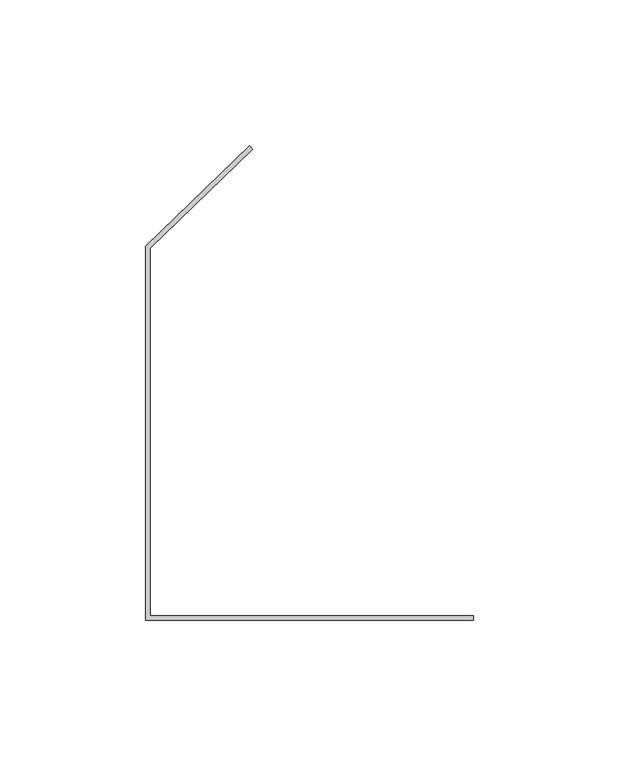
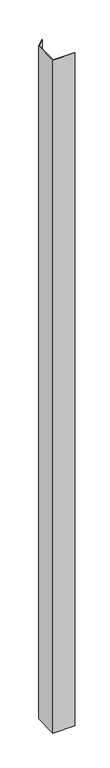
"""IFC4 building model written with IfcOpenShell, lengths in millimetres: proxy geometry, Generic Models 11:Generic Models 1:306267:Generic Models 1:306267 : Generic Models 11:Generic Models 1:306267:300405:Generic Models 1:306267:Generic Models 1:306267 : Generic Models 11:Generic Models 1:306267:300405 : Generic Models 11:Generic Models 1:306267:Generic Models 1:306267 : Generic Models 11:Generic Models 1:306267:300405:22 : Generic Models 11:Generic Models 1:306267:Generic Models 1:306267 : Generic Models 11:Generic Models 1:306267:300405:Generic Models 1:306267:Generic Models 1:306267 : Generic Models 11:Generic Models 1:306267:300405 : Generic Models 11:Generic Models 1:306267:Generic Models 1:306267 : Generic Models 11:Generic Models 1:306267:300405:300182."""

from ifc_helpers import new_model, si_unit, frame, origin, place, context, project, spatial, polyline, outline, extrude, source, transform, mapped, element, save


def generic_models_ad167b78(model_context):
    return source(origin(), model_context, "Body", "SweptSolid", [
        extrude(outline(polyline([(578579.828326, -568246.7263189), (578579.828326, -568118.5331318), (578615.3859082, -568084.0659821), (578616.5085764, -568085.1886502), (578581.415826, -568119.2052228), (578581.415826, -568245.1388189), (578692.2171387, -568245.1388189), (578692.2171387, -568246.7263189), (578579.828326, -568246.7263189)])), frame((0.0, 0.0, 4853.797603), z_axis=(0.0, 0.0, 1.0), x_axis=(1.0, 0.0, 0.0)), (0.0, 0.0, 1.0), 3695.7),
    ])


if __name__ == "__main__":
    model = new_model("IFC4")
    model_context = context("Model", 3, world=origin())
    ifc_project = project(units=[si_unit("LENGTHUNIT", "METRE", prefix="MILLI")], contexts=[model_context])
    site = spatial("IfcSite", under=ifc_project)
    building = spatial("IfcBuilding", under=site)
    placement = place(None, origin())
    generic_models_shape = generic_models_ad167b78(model_context)
    element("IfcBuildingElementProxy", 1, Name="Generic Models 11:Generic Models 1:306267:Generic Models 1:306267 : Generic Models 11:Generic Models 1:306267:300405:Generic Models 1:306267:Generic Models 1:306267 : Generic Models 11:Generic Models 1:306267:300405 : Generic Models 11:Generic Models 1:306267:Generic Models 1:306267 : Generic Models 11:Generic Models 1:306267:300405:22 : Generic Models 11:Generic Models 1:306267:Generic Models 1:306267 : Generic Models 11:Generic Models 1:306267:300405:Generic Models 1:306267:Generic Models 1:306267 : Generic Models 11:Generic Models 1:306267:300405 : Generic Models 11:Generic Models 1:306267:Generic Models 1:306267 : Generic Models 11:Generic Models 1:306267:300405:300182", ObjectType="Generic Models 11:Generic Models 1:306267:Generic Models 1:306267 : Generic Models 11:Generic Models 1:306267:300405:Generic Models 1:306267:Generic Models 1:306267 : Generic Models 11:Generic Models 1:306267:300405 : Generic Models 11:Generic Models 1:306267:Generic Models 1:306267 : Generic Models 11:Generic Models 1:306267:300405:22 : Generic Models 11:Generic Models 1:306267:Generic Models 1:306267 : Generic Models 11:Generic Models 1:306267:300405:Generic Models 1:306267:Generic Models 1:306267 : Generic Models 11:Generic Models 1:306267:300405 : Generic Models 11:Generic Models 1:306267:Generic Models 1:306267 : Generic Models 11:Generic Models 1:306267:300405:300182", at=placement, inside=building, context=model_context, shape_type="MappedRepresentation", body=[
        mapped(generic_models_shape, transform((0.0, 0.0, 0.0), x_axis=(1.0, 0.0, 0.0), y_axis=(0.0, 1.0, 0.0), z_axis=(0.0, 0.0, 1.0))),
    ])
    save(model, "model.ifc")

# Revit data of these elements
# Type "Generic Models 11:Generic Models 1:306267:Generic Models 1:306267 : Generic Models 11:Generic Models 1:306267:300405:Generic Models 1:306267:Generic Models 1:306267 : Generic Models 11:Generic Models 1:306267:300405 : Generic Models 11:Generic Models 1:306267:Generic Models 1:306267 : Generic Models 11:Generic Models 1:306267:300405:22 : Generic Models 11:Generic Models 1:306267:Generic Models 1:306267 : Generic Models 11:Generic Models 1:306267:300405:Generic Models 1:306267:Generic Models 1:306267 : Generic Models 11:Generic Models 1:306267:300405 : Generic Models 11:Generic Models 1:306267:Generic Models 1:306267 : Generic Models 11:Generic Models 1:306267:300405:300182"
#   NameOverride = "Generic Models 11:Generic Models 1:306267:Generic Models 1:306267 : Generic Models 11:Generic Models 1:306267:300405:Generic Models 1:306267:Generic Models 1:306267 : Generic Models 11:Generic Models 1:306267:300405 : Generic Models 11:Generic Models 1:306267:Generic Models 1:306267 : Generic Models 11:Generic Models 1:306267:300405:300182"
#   ObjectTypeOverride = "Generic Models 1:306267:Generic Models 1:306267 : Generic Models 11:Generic Models 1:306267:300405 : Generic Models 11:Generic Models 1:306267:Generic Models 1:306267 : Generic Models 11:Generic Models 1:306267:300405"
#   Reference = "Generic Models 1"
#   Tag = "300182"
# Element 1 (IfcBuildingElementProxy, "Generic Models 11:Generic Models 1:306267:Generic Models 1:306267 : Generic Models 11:Generic Models 1:306267:300405:Generic Models 1:306267:Generic Models 1:306267 : Generic Models 11:Generic Models 1:306267:300405 : Generic Models 11:Generic Models 1:306267:Generic Models 1:306267 : Generic Models 11:Generic Models 1:306267:300405:22 : Generic Models 11:Generic Models 1:306267:Generic Models 1:306267 : Generic Models 11:Generic Models 1:306267:300405:Generic Models 1:306267:Generic Models 1:306267 : Generic Models 11:Generic Models 1:306267:300405 : Generic Models 11:Generic Models 1:306267:Generic Models 1:306267 : Generic Models 11:Generic Models 1:306267:300405:300182")
#   Materials on its faces: "BRAKE METAL CLOSURE TRIM"
# Materials
#   "BRAKE METAL CLOSURE TRIM": class "Unassigned", colour RGB 182 182 182, transparency 0, Cost = 0
